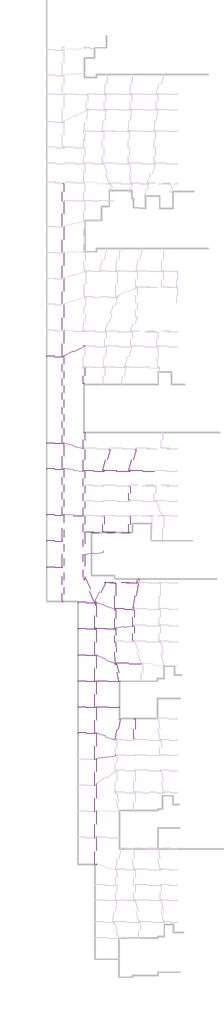
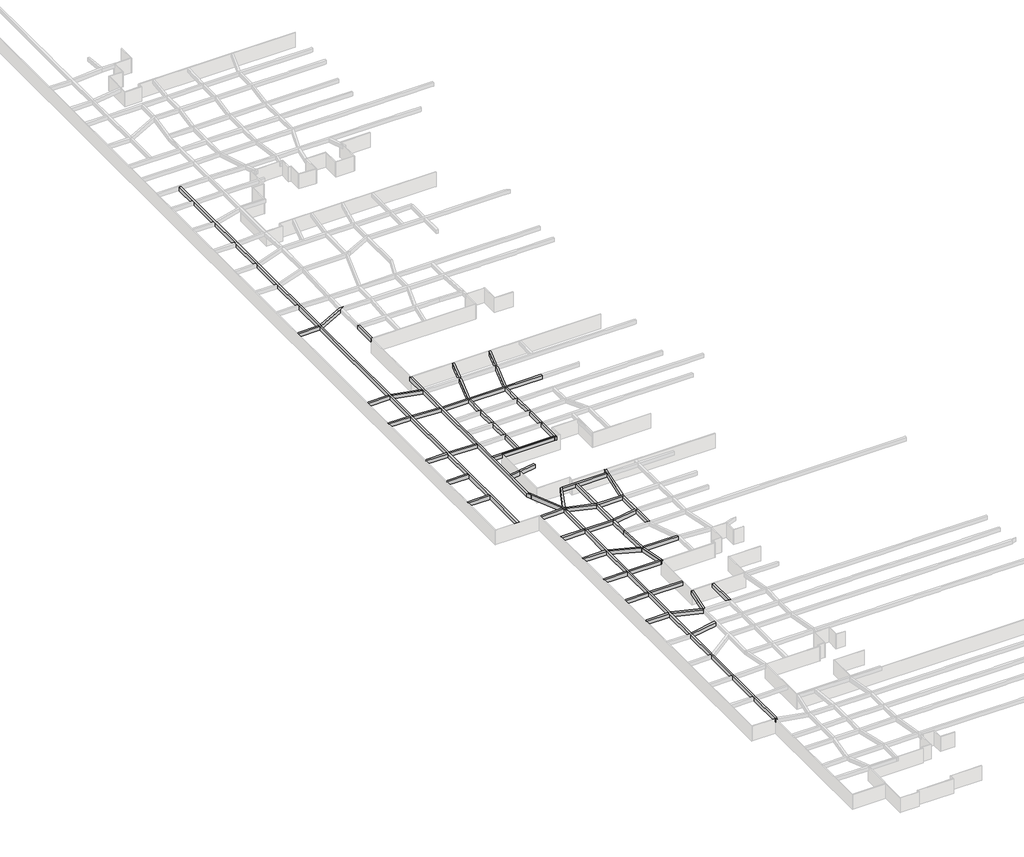
# One storey, part 14 of 45: 52 beams.
"""IFC4 building model written with IfcOpenShell, lengths in millimetres."""

from ifc_helpers import new_model, si_unit, frame, origin, place, context, project, spatial, polyline, outline, extrude, faceted_brep, element, save

model = new_model("IFC4")

# Units and contexts
model_context = context("Model", 3, world=origin())
ifc_project = project(units=[si_unit("LENGTHUNIT", "METRE", prefix="MILLI")], contexts=[model_context])

# Site, building, storey
site = spatial("IfcSite", under=ifc_project)
building = spatial("IfcBuilding", under=site)
storey = spatial("IfcBuildingStorey", under=building, Name="户型图", Elevation=0.0)

# Beams
placement = place(None, origin())
element("IfcBeam", 1, ObjectType="混凝土 - 矩形梁 : KL_beam", at=placement, inside=storey, context=model_context, shape_type="Brep", body=[
    faceted_brep([(-149959.8528414, -79527.7310375, 3300.0), (-150359.8528414, -79527.7310375, 3300.0), (-150359.8528414, -79527.7310375, 2500.0), (-149959.8528414, -79527.7310375, 2500.0), (-149959.8528414, -53780.5235569, 3300.0), (-149959.8528414, -53380.2797392, 3300.0), (-149959.8528414, -40042.1213562, 3300.0), (-149959.8528414, -39640.5934211, 3300.0), (-149959.8528414, -32335.6164347, 3300.0), (-149959.8528414, -31923.370983, 3300.0), (-149959.8528414, -6268.0099062, 3300.0), (-149959.8528414, -5819.0794111, 3300.0), (-149959.8528414, 1447.4441887, 3300.0), (-149959.8528414, 1847.6880064, 3300.0), (-149959.8528414, 9311.8916379, 3300.0), (-149959.8528414, 9734.9399104, 3300.0), (-149959.8528414, 17012.0067836, 3300.0), (-149959.8528414, 17435.0550561, 3300.0), (-149959.8528414, 24766.7995471, 3300.0), (-149959.8528414, 25167.5987199, 3300.0), (-149959.8528414, 32603.9353313, 3300.0), (-149959.8528414, 33020.0551056, 3300.0), (-149959.8528414, 40354.5502515, 3300.0), (-149959.8528414, 40754.5502515, 3300.0), (-149959.8528414, 45854.5502515, 3300.0), (-150359.8528414, 45854.5502515, 3300.0), (-150359.8528414, 40754.5502515, 3300.0), (-150359.8528414, 40354.5502515, 3300.0), (-150359.8528414, 32954.5502515, 3300.0), (-150359.8528414, 32554.5502515, 3300.0), (-150359.8528414, 25154.5502515, 3300.0), (-150359.8528414, 24754.5502515, 3300.0), (-150359.8528414, 17354.5502515, 3300.0), (-150359.8528414, 16954.5502515, 3300.0), (-150359.8528414, 9654.5502515, 3300.0), (-150359.8528414, 9254.5502515, 3300.0), (-150359.8528414, 1854.5502515, 3300.0), (-150359.8528414, 1454.5502515, 3300.0), (-150359.8528414, -5945.4497485, 3300.0), (-150359.8528414, -6345.4497485, 3300.0), (-150359.8528414, -31879.6281083, 3300.0), (-150359.8528414, -32279.6281083, 3300.0), (-150359.8528414, -39623.8596559, 3300.0), (-150359.8528414, -40023.8596559, 3300.0), (-150359.8528414, -53373.4174942, 3300.0), (-150359.8528414, -53773.4174942, 3300.0), (-150359.8528414, -61189.4871623, 3300.0), (-150359.8528414, -61589.4871623, 3300.0), (-150359.8528414, -69027.7310375, 3300.0), (-150359.8528414, -69427.7310375, 3300.0), (-150359.8528414, 45854.5502515, 2500.0), (-150359.8528414, 40754.5502515, 2500.0), (-150359.8528414, 40354.5502515, 2500.0), (-150359.8528414, 32954.5502515, 2500.0), (-150359.8528414, 32554.5502515, 2500.0), (-150359.8528414, 25154.5502515, 2500.0), (-150359.8528414, 24754.5502515, 2500.0), (-150359.8528414, 17354.5502515, 2500.0), (-150359.8528414, 16954.5502515, 2500.0), (-150359.8528414, 9654.5502515, 2500.0), (-150359.8528414, 9254.5502515, 2500.0), (-150359.8528414, 1854.5502515, 2500.0), (-150359.8528414, 1454.5502515, 2500.0), (-150359.8528414, -5945.4497485, 2500.0), (-150359.8528414, -6345.4497485, 2500.0), (-150359.8528414, -31879.6281083, 2500.0), (-150359.8528414, -32279.6281083, 2500.0), (-150359.8528414, -39623.8596559, 2500.0), (-150359.8528414, -40023.8596559, 2500.0), (-150359.8528414, -53373.4174942, 2500.0), (-150359.8528414, -53773.4174942, 2500.0), (-150359.8528414, -61189.4871623, 2500.0), (-150359.8528414, -61589.4871623, 2500.0), (-150359.8528414, -69027.7310375, 2500.0), (-150359.8528414, -69427.7310375, 2500.0), (-149959.8528414, 45854.5502515, 2500.0), (-149959.8528414, 40754.5502515, 2500.0), (-149959.8528414, 40354.5502515, 2500.0), (-149959.8528414, 33020.0551056, 2500.0), (-149959.8528414, 32603.9353313, 2500.0), (-149959.8528414, 25167.5987199, 2500.0), (-149959.8528414, 24766.7995471, 2500.0), (-149959.8528414, 17435.0550561, 2500.0), (-149959.8528414, 17012.0067836, 2500.0), (-149959.8528414, 9734.9399104, 2500.0), (-149959.8528414, 9311.8916379, 2500.0), (-149959.8528414, 1847.6880064, 2500.0), (-149959.8528414, 1447.4441887, 2500.0), (-149959.8528414, -5819.0794111, 2500.0), (-149959.8528414, -6268.0099062, 2500.0), (-149959.8528414, -31923.370983, 2500.0), (-149959.8528414, -32335.6164347, 2500.0), (-149959.8528414, -39640.5934211, 2500.0), (-149959.8528414, -40042.1213562, 2500.0), (-149959.8528414, -53380.2797392, 2500.0), (-149959.8528414, -53780.5235569, 2500.0)], [[[0, 1, 2, 3]], [[1, 0, 4, 5, 6, 7, 8, 9, 10, 11, 12, 13, 14, 15, 16, 17, 18, 19, 20, 21, 22, 23, 24, 25, 26, 27, 28, 29, 30, 31, 32, 33, 34, 35, 36, 37, 38, 39, 40, 41, 42, 43, 44, 45, 46, 47, 48, 49]], [[2, 1, 49, 48, 47, 46, 45, 44, 43, 42, 41, 40, 39, 38, 37, 36, 35, 34, 33, 32, 31, 30, 29, 28, 27, 26, 25, 50, 51, 52, 53, 54, 55, 56, 57, 58, 59, 60, 61, 62, 63, 64, 65, 66, 67, 68, 69, 70, 71, 72, 73, 74]], [[3, 2, 74, 73, 72, 71, 70, 69, 68, 67, 66, 65, 64, 63, 62, 61, 60, 59, 58, 57, 56, 55, 54, 53, 52, 51, 50, 75, 76, 77, 78, 79, 80, 81, 82, 83, 84, 85, 86, 87, 88, 89, 90, 91, 92, 93, 94, 95]], [[0, 3, 95, 94, 93, 92, 91, 90, 89, 88, 87, 86, 85, 84, 83, 82, 81, 80, 79, 78, 77, 76, 75, 24, 23, 22, 21, 20, 19, 18, 17, 16, 15, 14, 13, 12, 11, 10, 9, 8, 7, 6, 5, 4]], [[25, 24, 75, 50]]]),
])
element("IfcBeam", 2, ObjectType="混凝土 - 矩形梁 : KL_beam", at=placement, inside=storey, context=model_context, shape_type="SweptSolid", body=[
    extrude(outline(polyline([(-155040.1872489, -6345.4497485), (-155040.1872489, -5945.4497485), (-150359.8528414, -5945.4497485), (-150359.8528414, -6345.4497485), (-155040.1872489, -6345.4497485)])), frame((0.0, 0.0, 2500.0), z_axis=(0.0, 0.0, 1.0), x_axis=(1.0, 0.0, 0.0)), (0.0, 0.0, 1.0), 800.0),
])
element("IfcBeam", 3, ObjectType="混凝土 - 矩形梁 : KL_beam", at=placement, inside=storey, context=model_context, shape_type="Brep", body=[
    faceted_brep([(-143362.5840071, -2906.533538, 3300.0), (-143704.0852782, -2906.533538, 3300.0), (-144104.0852782, -2906.533538, 3300.0), (-144243.659713, -2906.533538, 3300.0), (-149959.8528414, -5819.0794111, 3300.0), (-149959.8528414, -6268.0099062, 3300.0), (-144147.6282093, -3306.533538, 3300.0), (-143362.5840071, -2906.533538, 2500.0), (-149959.8528414, -6268.0099062, 2500.0), (-144147.6282093, -3306.533538, 2500.0), (-144243.659713, -2906.533538, 2500.0), (-144104.0852782, -2906.533538, 2500.0), (-143704.0852782, -2906.533538, 2500.0), (-149959.8528414, -5819.0794111, 2500.0)], [[[0, 1, 2, 3, 4, 5, 6]], [[7, 0, 6, 5, 8, 9]], [[10, 11, 12, 7, 9, 8, 13]], [[3, 10, 13, 4]], [[5, 4, 13, 8]], [[3, 2, 1, 0, 7, 12, 11, 10]]]),
])
element("IfcBeam", 4, ObjectType="混凝土 - 矩形梁 : KL_beam", at=placement, inside=storey, context=model_context, shape_type="SweptSolid", body=[
    extrude(outline(polyline([(-143704.0852782, -14343.8680223), (-144104.0852782, -14343.8680223), (-144104.0852782, -9543.8680223), (-143704.0852782, -9543.8680223), (-143704.0852782, -14343.8680223)])), frame((0.0, 0.0, 2500.0), z_axis=(0.0, 0.0, 1.0), x_axis=(1.0, 0.0, 0.0)), (0.0, 0.0, 1.0), 800.0),
])
element("IfcBeam", 5, ObjectType="混凝土 - 矩形梁 : KL_beam", at=placement, inside=storey, context=model_context, shape_type="Brep", body=[
    faceted_brep([(-122515.2422867, -40570.1922876, 3300.0), (-122515.2422867, -40170.1922876, 3300.0), (-130022.2070751, -40170.1922876, 3300.0), (-130438.3268494, -40170.1922876, 3300.0), (-137822.2070751, -40170.1922876, 3300.0), (-138238.3268494, -40170.1922876, 3300.0), (-143687.6160394, -40170.1922876, 3300.0), (-143687.6160394, -40570.1922876, 3300.0), (-138287.6160394, -40570.1922876, 3300.0), (-137887.6160394, -40570.1922876, 3300.0), (-130487.6160394, -40570.1922876, 3300.0), (-130087.6160394, -40570.1922876, 3300.0), (-122515.2422867, -40570.1922876, 2500.0), (-143687.6160394, -40570.1922876, 2500.0), (-138287.6160394, -40570.1922876, 2500.0), (-137887.6160394, -40570.1922876, 2500.0), (-130487.6160394, -40570.1922876, 2500.0), (-130087.6160394, -40570.1922876, 2500.0), (-122515.2422867, -40170.1922876, 2500.0), (-143687.6160394, -40170.1922876, 2500.0), (-138238.3268494, -40170.1922876, 2500.0), (-137822.2070751, -40170.1922876, 2500.0), (-130438.3268494, -40170.1922876, 2500.0), (-130022.2070751, -40170.1922876, 2500.0)], [[[0, 1, 2, 3, 4, 5, 6, 7, 8, 9, 10, 11]], [[12, 0, 11, 10, 9, 8, 7, 13, 14, 15, 16, 17]], [[18, 12, 17, 16, 15, 14, 13, 19, 20, 21, 22, 23]], [[1, 18, 23, 22, 21, 20, 19, 6, 5, 4, 3, 2]], [[1, 0, 12, 18]], [[7, 6, 19, 13]]]),
])
element("IfcBeam", 6, ObjectType="混凝土 - 矩形梁 : KL_beam", at=placement, inside=storey, context=model_context, shape_type="SweptSolid", body=[
    extrude(outline(polyline([(-144087.6160394, -33387.4840571), (-144087.6160394, -33799.7295088), (-149959.8528414, -32335.6164347), (-149959.8528414, -31923.370983), (-144087.6160394, -33387.4840571)])), frame((0.0, 0.0, 2500.0), z_axis=(0.0, 0.0, 1.0), x_axis=(1.0, 0.0, 0.0)), (0.0, 0.0, 1.0), 800.0),
])
element("IfcBeam", 7, ObjectType="混凝土 - 矩形梁 : KL_beam", at=placement, inside=storey, context=model_context, shape_type="SweptSolid", body=[
    extrude(outline(polyline([(-155040.1872489, -32279.6281083), (-155040.1872489, -31879.6281083), (-150359.8528414, -31879.6281083), (-150359.8528414, -32279.6281083), (-155040.1872489, -32279.6281083)])), frame((0.0, 0.0, 2500.0), z_axis=(0.0, 0.0, 1.0), x_axis=(1.0, 0.0, 0.0)), (0.0, 0.0, 1.0), 800.0),
])
element("IfcBeam", 8, ObjectType="混凝土 - 矩形梁 : KL_beam", at=placement, inside=storey, context=model_context, shape_type="SweptSolid", body=[
    extrude(outline(polyline([(-144087.6160394, -40154.3475708), (-144087.6160394, -40555.8755059), (-149959.8528414, -40042.1213562), (-149959.8528414, -39640.5934211), (-144087.6160394, -40154.3475708)])), frame((0.0, 0.0, 2500.0), z_axis=(0.0, 0.0, 1.0), x_axis=(1.0, 0.0, 0.0)), (0.0, 0.0, 1.0), 800.0),
])
element("IfcBeam", 9, ObjectType="混凝土 - 矩形梁 : KL_beam", at=placement, inside=storey, context=model_context, shape_type="SweptSolid", body=[
    extrude(outline(polyline([(-155040.1872489, -40023.8596559), (-155040.1872489, -39623.8596559), (-150359.8528414, -39623.8596559), (-150359.8528414, -40023.8596559), (-155040.1872489, -40023.8596559)])), frame((0.0, 0.0, 2500.0), z_axis=(0.0, 0.0, 1.0), x_axis=(1.0, 0.0, 0.0)), (0.0, 0.0, 1.0), 800.0),
])
element("IfcBeam", 10, ObjectType="混凝土 - 矩形梁 : KL_beam", at=placement, inside=storey, context=model_context, shape_type="SweptSolid", body=[
    extrude(outline(polyline([(-149959.8528414, -53780.5235569), (-149959.8528414, -53380.2797392), (-144087.6160394, -53585.342767), (-144087.6160394, -53985.5865847), (-149959.8528414, -53780.5235569)])), frame((0.0, 0.0, 2500.0), z_axis=(0.0, 0.0, 1.0), x_axis=(1.0, 0.0, 0.0)), (0.0, 0.0, 1.0), 800.0),
])
element("IfcBeam", 11, ObjectType="混凝土 - 矩形梁 : KL_beam", at=placement, inside=storey, context=model_context, shape_type="SweptSolid", body=[
    extrude(outline(polyline([(-155040.1872489, -53773.4174942), (-155040.1872489, -53373.4174942), (-150359.8528414, -53373.4174942), (-150359.8528414, -53773.4174942), (-155040.1872489, -53773.4174942)])), frame((0.0, 0.0, 2500.0), z_axis=(0.0, 0.0, 1.0), x_axis=(1.0, 0.0, 0.0)), (0.0, 0.0, 1.0), 800.0),
])
element("IfcBeam", 12, ObjectType="混凝土 - 矩形梁 : KL_beam", at=placement, inside=storey, context=model_context, shape_type="SweptSolid", body=[
    extrude(outline(polyline([(-155040.1872489, -61589.4871623), (-155040.1872489, -61189.4871623), (-150359.8528414, -61189.4871623), (-150359.8528414, -61589.4871623), (-155040.1872489, -61589.4871623)])), frame((0.0, 0.0, 2500.0), z_axis=(0.0, 0.0, 1.0), x_axis=(1.0, 0.0, 0.0)), (0.0, 0.0, 1.0), 800.0),
])
element("IfcBeam", 13, ObjectType="混凝土 - 矩形梁 : KL_beam", at=placement, inside=storey, context=model_context, shape_type="SweptSolid", body=[
    extrude(outline(polyline([(-155040.1872489, -69427.7310375), (-155040.1872489, -69027.7310375), (-150359.8528414, -69027.7310375), (-150359.8528414, -69427.7310375), (-155040.1872489, -69427.7310375)])), frame((0.0, 0.0, 2500.0), z_axis=(0.0, 0.0, 1.0), x_axis=(1.0, 0.0, 0.0)), (0.0, 0.0, 1.0), 800.0),
])
element("IfcBeam", 14, ObjectType="混凝土 - 矩形梁 : KL_beam", at=placement, inside=storey, context=model_context, shape_type="Brep", body=[
    faceted_brep([(-143687.6160394, -28841.7316236, 3300.0), (-143687.6160394, -28841.7316236, 2500.0), (-144087.6160394, -28841.7316236, 2500.0), (-144087.6160394, -28841.7316236, 3300.0), (-144087.6160394, -33387.4840571, 3300.0), (-144087.6160394, -33799.7295088, 3300.0), (-144087.6160394, -40154.3475708, 3300.0), (-144087.6160394, -40555.8755059, 3300.0), (-144087.6160394, -53585.342767, 3300.0), (-144087.6160394, -53985.5865847, 3300.0), (-144087.6160394, -72184.2429359, 3300.0), (-143687.6160394, -73082.6576455, 3300.0), (-143687.6160394, -72099.2203112, 3300.0), (-143687.6160394, -65809.5515498, 3300.0), (-143687.6160394, -65403.3809051, 3300.0), (-143687.6160394, -58989.4871623, 3300.0), (-143687.6160394, -58589.4871623, 3300.0), (-143687.6160394, -53989.4871623, 3300.0), (-143687.6160394, -53589.4871623, 3300.0), (-143687.6160394, -49549.7368283, 3300.0), (-143687.6160394, -49149.7368283, 3300.0), (-143687.6160394, -44984.7380181, 3300.0), (-143687.6160394, -44584.7380181, 3300.0), (-143687.6160394, -40570.1922876, 3300.0), (-143687.6160394, -40170.1922876, 3300.0), (-143687.6160394, -33842.9557231, 3300.0), (-143687.6160394, -33442.9557231, 3300.0), (-144087.6160394, -33387.4840571, 2500.0), (-144087.6160394, -33799.7295088, 2500.0), (-144087.6160394, -40154.3475708, 2500.0), (-144087.6160394, -40555.8755059, 2500.0), (-144087.6160394, -53585.342767, 2500.0), (-144087.6160394, -53985.5865847, 2500.0), (-144087.6160394, -72184.2429359, 2500.0), (-143687.6160394, -33442.9557231, 2500.0), (-143687.6160394, -33842.9557231, 2500.0), (-143687.6160394, -40170.1922876, 2500.0), (-143687.6160394, -40570.1922876, 2500.0), (-143687.6160394, -44584.7380181, 2500.0), (-143687.6160394, -44984.7380181, 2500.0), (-143687.6160394, -49149.7368283, 2500.0), (-143687.6160394, -49549.7368283, 2500.0), (-143687.6160394, -53589.4871623, 2500.0), (-143687.6160394, -53989.4871623, 2500.0), (-143687.6160394, -58589.4871623, 2500.0), (-143687.6160394, -58989.4871623, 2500.0), (-143687.6160394, -65403.3809051, 2500.0), (-143687.6160394, -65809.5515498, 2500.0), (-143687.6160394, -72099.2203112, 2500.0), (-143687.6160394, -73082.6576455, 2500.0)], [[[0, 1, 2, 3]], [[0, 3, 4, 5, 6, 7, 8, 9, 10, 11, 12, 13, 14, 15, 16, 17, 18, 19, 20, 21, 22, 23, 24, 25, 26]], [[3, 2, 27, 28, 29, 30, 31, 32, 33, 10, 9, 8, 7, 6, 5, 4]], [[2, 1, 34, 35, 36, 37, 38, 39, 40, 41, 42, 43, 44, 45, 46, 47, 48, 49, 33, 32, 31, 30, 29, 28, 27]], [[1, 0, 26, 25, 24, 23, 22, 21, 20, 19, 18, 17, 16, 15, 14, 13, 12, 11, 49, 48, 47, 46, 45, 44, 43, 42, 41, 40, 39, 38, 37, 36, 35, 34]], [[11, 10, 33, 49]]]),
])
element("IfcBeam", 15, ObjectType="混凝土 - 矩形梁 : KL_beam", at=placement, inside=storey, context=model_context, shape_type="Brep", body=[
    faceted_brep([(-140271.0282376, -80756.4394897, 3300.0), (-140271.0282376, -80088.1741567, 3300.0), (-140271.0282376, -79773.0021554, 3300.0), (-140324.9318597, -79651.9326379, 3300.0), (-140466.6372594, -79333.6570992, 3300.0), (-143687.6160394, -72099.2203112, 3300.0), (-143687.6160394, -73082.6576455, 3300.0), (-140778.9001436, -79615.7405122, 3300.0), (-140671.0282376, -79858.0247801, 3300.0), (-140271.0282376, -80756.4394897, 2500.0), (-143687.6160394, -73082.6576455, 2500.0), (-140778.9001436, -79615.7405122, 2500.0), (-140671.0282376, -79858.0247801, 2500.0), (-140271.0282376, -79773.0021554, 2500.0), (-140271.0282376, -80088.1741567, 2500.0), (-143687.6160394, -72099.2203112, 2500.0), (-140466.6372594, -79333.6570992, 2500.0), (-140324.9318597, -79651.9326379, 2500.0)], [[[0, 1, 2, 3, 4, 5, 6, 7, 8]], [[9, 0, 8, 7, 6, 10, 11, 12]], [[13, 14, 9, 12, 11, 10, 15, 16, 17]], [[2, 13, 17, 16, 15, 5, 4, 3]], [[6, 5, 15, 10]], [[2, 1, 0, 9, 14, 13]]]),
])
element("IfcBeam", 16, ObjectType="混凝土 - 矩形梁 : KL_beam", at=placement, inside=storey, context=model_context, shape_type="SweptSolid", body=[
    extrude(outline(polyline([(-138287.6160394, -40570.1922876), (-137887.6160394, -40570.1922876), (-137887.6160394, -44584.7380181), (-138287.6160394, -44584.7380181), (-138287.6160394, -40570.1922876)])), frame((0.0, 0.0, 2500.0), z_axis=(0.0, 0.0, 1.0), x_axis=(1.0, 0.0, 0.0)), (0.0, 0.0, 1.0), 800.0),
    extrude(outline(polyline([(-138287.6160394, -44984.7380181), (-137887.6160394, -44984.7380181), (-137887.6160394, -49149.7368283), (-138287.6160394, -49149.7368283), (-138287.6160394, -44984.7380181)])), frame((0.0, 0.0, 2500.0), z_axis=(0.0, 0.0, 1.0), x_axis=(1.0, 0.0, 0.0)), (0.0, 0.0, 1.0), 800.0),
    extrude(outline(polyline([(-138287.6160394, -49549.7368283), (-137887.6160394, -49549.7368283), (-137887.6160394, -53589.4871623), (-138287.6160394, -53589.4871623), (-138287.6160394, -49549.7368283)])), frame((0.0, 0.0, 2500.0), z_axis=(0.0, 0.0, 1.0), x_axis=(1.0, 0.0, 0.0)), (0.0, 0.0, 1.0), 800.0),
    extrude(outline(polyline([(-138287.6160394, -53989.4871623), (-137887.6160394, -53989.4871623), (-137887.6160394, -58589.4871623), (-138287.6160394, -58589.4871623), (-138287.6160394, -53989.4871623)])), frame((0.0, 0.0, 2500.0), z_axis=(0.0, 0.0, 1.0), x_axis=(1.0, 0.0, 0.0)), (0.0, 0.0, 1.0), 800.0),
])
element("IfcBeam", 17, ObjectType="混凝土 - 矩形梁 : KL_beam", at=placement, inside=storey, context=model_context, shape_type="SweptSolid", body=[
    extrude(outline(polyline([(-134969.1006355, -28769.0455688), (-134584.5959571, -28879.3005111), (-135893.2030313, -33442.9557231), (-136309.3228056, -33442.9557231), (-134969.1006355, -28769.0455688)])), frame((0.0, 0.0, 2500.0), z_axis=(0.0, 0.0, 1.0), x_axis=(1.0, 0.0, 0.0)), (0.0, 0.0, 1.0), 800.0),
    extrude(outline(polyline([(-136424.0209599, -33842.9557231), (-136007.9011856, -33842.9557231), (-137822.2070751, -40170.1922876), (-138238.3268494, -40170.1922876), (-136424.0209599, -33842.9557231)])), frame((0.0, 0.0, 2500.0), z_axis=(0.0, 0.0, 1.0), x_axis=(1.0, 0.0, 0.0)), (0.0, 0.0, 1.0), 800.0),
])
element("IfcBeam", 18, ObjectType="混凝土 - 矩形梁 : KL_beam", at=placement, inside=storey, context=model_context, shape_type="SweptSolid", body=[
    extrude(outline(polyline([(-127169.1006355, -28769.0455688), (-126784.5959571, -28879.3005111), (-128093.2030313, -33442.9557231), (-128509.3228056, -33442.9557231), (-127169.1006355, -28769.0455688)])), frame((0.0, 0.0, 2500.0), z_axis=(0.0, 0.0, 1.0), x_axis=(1.0, 0.0, 0.0)), (0.0, 0.0, 1.0), 800.0),
    extrude(outline(polyline([(-128624.0209599, -33842.9557231), (-128207.9011856, -33842.9557231), (-130022.2070751, -40170.1922876), (-130438.3268494, -40170.1922876), (-128624.0209599, -33842.9557231)])), frame((0.0, 0.0, 2500.0), z_axis=(0.0, 0.0, 1.0), x_axis=(1.0, 0.0, 0.0)), (0.0, 0.0, 1.0), 800.0),
])
element("IfcBeam", 19, ObjectType="混凝土 - 矩形梁 : KL_beam", at=placement, inside=storey, context=model_context, shape_type="SweptSolid", body=[
    extrude(outline(polyline([(-130487.6160394, -40570.1922876), (-130087.6160394, -40570.1922876), (-130087.6160394, -44584.7380181), (-130487.6160394, -44584.7380181), (-130487.6160394, -40570.1922876)])), frame((0.0, 0.0, 2500.0), z_axis=(0.0, 0.0, 1.0), x_axis=(1.0, 0.0, 0.0)), (0.0, 0.0, 1.0), 800.0),
    extrude(outline(polyline([(-130087.6160394, -53589.4871623), (-130487.6160394, -53589.4871623), (-130487.6160394, -49549.7368283), (-130087.6160394, -49549.7368283), (-130087.6160394, -53589.4871623)])), frame((0.0, 0.0, 2500.0), z_axis=(0.0, 0.0, 1.0), x_axis=(1.0, 0.0, 0.0)), (0.0, 0.0, 1.0), 800.0),
    extrude(outline(polyline([(-130487.6160394, -44984.7380181), (-130087.6160394, -44984.7380181), (-130087.6160394, -49149.7368283), (-130487.6160394, -49149.7368283), (-130487.6160394, -44984.7380181)])), frame((0.0, 0.0, 2500.0), z_axis=(0.0, 0.0, 1.0), x_axis=(1.0, 0.0, 0.0)), (0.0, 0.0, 1.0), 800.0),
])
element("IfcBeam", 20, ObjectType="混凝土 - 矩形梁 : KL_beam", at=placement, inside=storey, context=model_context, shape_type="Brep", body=[
    faceted_brep([(-130487.6160394, -58989.4871623, 3300.0), (-130087.6160394, -58989.4871623, 3300.0), (-130087.6160394, -53989.4871623, 3300.0), (-130487.6160394, -53989.4871623, 3300.0), (-130487.6160394, -58589.4871623, 3300.0), (-130487.6160394, -58989.4871623, 2500.0), (-130487.6160394, -53989.4871623, 2500.0), (-130487.6160394, -58589.4871623, 2500.0), (-130087.6160394, -58989.4871623, 2500.0), (-130087.6160394, -53989.4871623, 2500.0)], [[[0, 1, 2, 3, 4]], [[5, 0, 4, 3, 6, 7]], [[8, 5, 7, 6, 9]], [[1, 8, 9, 2]], [[3, 2, 9, 6]], [[1, 0, 5, 8]]]),
])
element("IfcBeam", 21, ObjectType="混凝土 - 矩形梁 : KL_beam", at=placement, inside=storey, context=model_context, shape_type="Brep", body=[
    faceted_brep([(-128818.6286131, -81886.7344834, 3300.0), (-128818.6286131, -81486.7344834, 3300.0), (-129189.4447502, -81486.7344834, 3300.0), (-134318.6286131, -81486.7344834, 3300.0), (-134488.0377959, -81486.7344834, 3300.0), (-134718.6286131, -81486.7344834, 3300.0), (-134718.6286131, -81833.5464328, 3300.0), (-134718.6286131, -81886.7344834, 3300.0), (-134318.6286131, -81886.7344834, 3300.0), (-129218.6286131, -81886.7344834, 3300.0), (-128818.6286131, -81886.7344834, 2500.0), (-134718.6286131, -81886.7344834, 2500.0), (-134318.6286131, -81886.7344834, 2500.0), (-129218.6286131, -81886.7344834, 2500.0), (-128818.6286131, -81486.7344834, 2500.0), (-134718.6286131, -81833.5464328, 2500.0), (-134718.6286131, -81486.7344834, 2500.0), (-134488.0377959, -81486.7344834, 2500.0), (-134318.6286131, -81486.7344834, 2500.0), (-129189.4447502, -81486.7344834, 2500.0)], [[[0, 1, 2, 3, 4, 5, 6, 7, 8, 9]], [[10, 0, 9, 8, 7, 11, 12, 13]], [[14, 10, 13, 12, 11, 15, 16, 17, 18, 19]], [[1, 14, 19, 18, 17, 16, 5, 4, 3, 2]], [[1, 0, 10, 14]], [[7, 6, 5, 16, 15, 11]]]),
])
element("IfcBeam", 22, ObjectType="混凝土 - 矩形梁 : KL_beam", at=placement, inside=storey, context=model_context, shape_type="Brep", body=[
    faceted_brep([(-129218.6286131, -86925.0852019, 3300.0), (-129001.1308804, -86886.7344834, 3300.0), (-128818.6286131, -86854.5544096, 3300.0), (-128818.6286131, -86486.7344834, 3300.0), (-128818.6286131, -81886.7344834, 3300.0), (-129218.6286131, -81886.7344834, 3300.0), (-129218.6286131, -86518.9145571, 3300.0), (-129218.6286131, -86925.0852019, 2500.0), (-129218.6286131, -81886.7344834, 2500.0), (-129218.6286131, -86518.9145571, 2500.0), (-128818.6286131, -86854.5544096, 2500.0), (-129001.1308804, -86886.7344834, 2500.0), (-128818.6286131, -81886.7344834, 2500.0), (-128818.6286131, -86486.7344834, 2500.0)], [[[0, 1, 2, 3, 4, 5, 6]], [[7, 0, 6, 5, 8, 9]], [[10, 11, 7, 9, 8, 12, 13]], [[2, 10, 13, 12, 4, 3]], [[5, 4, 12, 8]], [[2, 1, 0, 7, 11, 10]]]),
])
element("IfcBeam", 23, ObjectType="混凝土 - 矩形梁 : KL_beam", at=placement, inside=storey, context=model_context, shape_type="Brep", body=[
    faceted_brep([(-134452.5689874, -87441.7994605, 3300.0), (-134417.573522, -87841.7994605, 3300.0), (-134318.6286131, -87824.3528035, 3300.0), (-129218.6286131, -86925.0852019, 3300.0), (-129218.6286131, -86518.9145571, 3300.0), (-134318.6286131, -87418.1821587, 3300.0), (-134452.5689874, -87441.7994605, 2500.0), (-129218.6286131, -86518.9145571, 2500.0), (-134318.6286131, -87418.1821587, 2500.0), (-134417.573522, -87841.7994605, 2500.0), (-129218.6286131, -86925.0852019, 2500.0), (-134318.6286131, -87824.3528035, 2500.0)], [[[0, 1, 2, 3, 4, 5]], [[6, 0, 5, 4, 7, 8]], [[9, 6, 8, 7, 10, 11]], [[1, 9, 11, 10, 3, 2]], [[4, 3, 10, 7]], [[1, 0, 6, 9]]]),
])
element("IfcBeam", 24, ObjectType="混凝土 - 矩形梁 : KL_beam", at=placement, inside=storey, context=model_context, shape_type="Brep", body=[
    faceted_brep([(-134417.573522, -87841.7994605, 3300.0), (-134452.5689874, -87441.7994605, 3300.0), (-134718.6286131, -87441.7994605, 3300.0), (-140271.0282376, -87441.7994605, 3300.0), (-140635.0712547, -87441.7994605, 3300.0), (-140635.0712547, -87841.7994605, 3300.0), (-140235.0712547, -87841.7994605, 3300.0), (-134718.6286131, -87841.7994605, 3300.0), (-134452.5689874, -87441.7994605, 2500.0), (-134718.6286131, -87441.7994605, 2500.0), (-140271.0282376, -87441.7994605, 2500.0), (-140635.0712547, -87441.7994605, 2500.0), (-134417.573522, -87841.7994605, 2500.0), (-134718.6286131, -87841.7994605, 2500.0), (-140235.0712547, -87841.7994605, 2500.0), (-140635.0712547, -87841.7994605, 2500.0)], [[[0, 1, 2, 3, 4, 5, 6, 7]], [[1, 8, 9, 10, 11, 4, 3, 2]], [[8, 12, 13, 14, 15, 11, 10, 9]], [[12, 0, 7, 6, 5, 15, 14, 13]], [[0, 12, 8, 1]], [[5, 4, 11, 15]]]),
])
element("IfcBeam", 25, ObjectType="混凝土 - 矩形梁 : KL_beam", at=placement, inside=storey, context=model_context, shape_type="SweptSolid", body=[
    extrude(outline(polyline([(-134718.6286131, -81886.7344834), (-134318.6286131, -81886.7344834), (-134318.6286131, -87418.1821587), (-134452.5689874, -87441.7994605), (-134718.6286131, -87441.7994605), (-134718.6286131, -81886.7344834)])), frame((0.0, 0.0, 2500.0), z_axis=(0.0, 0.0, 1.0), x_axis=(1.0, 0.0, 0.0)), (0.0, 0.0, 1.0), 800.0),
])
element("IfcBeam", 26, ObjectType="混凝土 - 矩形梁 : KL_beam", at=placement, inside=storey, context=model_context, shape_type="Brep", body=[
    faceted_brep([(-134417.573522, -87841.7994605, 3300.0), (-134718.6286131, -87841.7994605, 3300.0), (-134718.6286131, -91641.7669719, 3300.0), (-134711.7663681, -91641.7669719, 3300.0), (-134318.6286131, -91641.7669719, 3300.0), (-134318.6286131, -91241.7669719, 3300.0), (-134318.6286131, -87824.3528035, 3300.0), (-134718.6286131, -87841.7994605, 2500.0), (-134718.6286131, -91641.7669719, 2500.0), (-134417.573522, -87841.7994605, 2500.0), (-134318.6286131, -87824.3528035, 2500.0), (-134318.6286131, -91241.7669719, 2500.0), (-134318.6286131, -91641.7669719, 2500.0), (-134711.7663681, -91641.7669719, 2500.0)], [[[0, 1, 2, 3, 4, 5, 6]], [[1, 7, 8, 2]], [[7, 9, 10, 11, 12, 13, 8]], [[10, 6, 5, 4, 12, 11]], [[1, 0, 9, 7]], [[0, 6, 10, 9]], [[4, 3, 2, 8, 13, 12]]]),
])
element("IfcBeam", 27, ObjectType="混凝土 - 矩形梁 : KL_beam", at=placement, inside=storey, context=model_context, shape_type="Brep", body=[
    faceted_brep([(-140635.0712547, -158399.1295185, 3300.0), (-140235.0712547, -158496.0420414, 3300.0), (-140235.0712547, -158084.4694025, 3300.0), (-140235.0712547, -150329.5553627, 3300.0), (-140235.0712547, -149929.5553627, 3300.0), (-140235.0712547, -142522.6839278, 3300.0), (-140235.0712547, -142122.4401101, 3300.0), (-140235.0712547, -134607.1099192, 3300.0), (-140235.0712547, -134112.6827282, 3300.0), (-140235.0712547, -126910.8224065, 3300.0), (-140235.0712547, -126503.1705503, 3300.0), (-140235.0712547, -119155.7020829, 3300.0), (-140235.0712547, -118732.7040614, 3300.0), (-140235.0712547, -111375.3373066, 3300.0), (-140235.0712547, -110975.3373066, 3300.0), (-140235.0712547, -103575.0953667, 3300.0), (-140235.0712547, -103175.0953667, 3300.0), (-140235.0712547, -95870.908911, 3300.0), (-140235.0712547, -95440.0063093, 3300.0), (-140235.0712547, -87841.7994605, 3300.0), (-140635.0712547, -87841.7994605, 3300.0), (-140635.0712547, -95375.3373066, 3300.0), (-140635.0712547, -95775.3373066, 3300.0), (-140635.0712547, -103175.3373066, 3300.0), (-140635.0712547, -103575.3373066, 3300.0), (-140635.0712547, -110975.3373066, 3300.0), (-140635.0712547, -111375.3373066, 3300.0), (-140635.0712547, -118675.3373066, 3300.0), (-140635.0712547, -119075.3373066, 3300.0), (-140635.0712547, -126546.3745528, 3300.0), (-140635.0712547, -126946.3745528, 3300.0), (-140635.0712547, -134305.27306, 3300.0), (-140635.0712547, -134705.27306, 3300.0), (-140635.0712547, -142129.5553627, 3300.0), (-140635.0712547, -142529.5553627, 3300.0), (-140635.0712547, -149929.5553627, 3300.0), (-140635.0712547, -150329.5553627, 3300.0), (-140635.0712547, -158399.1295185, 2500.0), (-140635.0712547, -87841.7994605, 2500.0), (-140635.0712547, -95375.3373066, 2500.0), (-140635.0712547, -95775.3373066, 2500.0), (-140635.0712547, -103175.3373066, 2500.0), (-140635.0712547, -103575.3373066, 2500.0), (-140635.0712547, -110975.3373066, 2500.0), (-140635.0712547, -111375.3373066, 2500.0), (-140635.0712547, -118675.3373066, 2500.0), (-140635.0712547, -119075.3373066, 2500.0), (-140635.0712547, -126546.3745528, 2500.0), (-140635.0712547, -126946.3745528, 2500.0), (-140635.0712547, -134305.27306, 2500.0), (-140635.0712547, -134705.27306, 2500.0), (-140635.0712547, -142129.5553627, 2500.0), (-140635.0712547, -142529.5553627, 2500.0), (-140635.0712547, -149929.5553627, 2500.0), (-140635.0712547, -150329.5553627, 2500.0), (-140235.0712547, -158496.0420414, 2500.0), (-140235.0712547, -87841.7994605, 2500.0), (-140235.0712547, -95440.0063093, 2500.0), (-140235.0712547, -95870.908911, 2500.0), (-140235.0712547, -103175.0953667, 2500.0), (-140235.0712547, -103575.0953667, 2500.0), (-140235.0712547, -110975.3373066, 2500.0), (-140235.0712547, -111375.3373066, 2500.0), (-140235.0712547, -118732.7040614, 2500.0), (-140235.0712547, -119155.7020829, 2500.0), (-140235.0712547, -126503.1705503, 2500.0), (-140235.0712547, -126910.8224065, 2500.0), (-140235.0712547, -134112.6827282, 2500.0), (-140235.0712547, -134607.1099192, 2500.0), (-140235.0712547, -142122.4401101, 2500.0), (-140235.0712547, -142522.6839278, 2500.0), (-140235.0712547, -149929.5553627, 2500.0), (-140235.0712547, -150329.5553627, 2500.0), (-140235.0712547, -158084.4694025, 2500.0)], [[[0, 1, 2, 3, 4, 5, 6, 7, 8, 9, 10, 11, 12, 13, 14, 15, 16, 17, 18, 19, 20, 21, 22, 23, 24, 25, 26, 27, 28, 29, 30, 31, 32, 33, 34, 35, 36]], [[37, 0, 36, 35, 34, 33, 32, 31, 30, 29, 28, 27, 26, 25, 24, 23, 22, 21, 20, 38, 39, 40, 41, 42, 43, 44, 45, 46, 47, 48, 49, 50, 51, 52, 53, 54]], [[55, 37, 54, 53, 52, 51, 50, 49, 48, 47, 46, 45, 44, 43, 42, 41, 40, 39, 38, 56, 57, 58, 59, 60, 61, 62, 63, 64, 65, 66, 67, 68, 69, 70, 71, 72, 73]], [[1, 55, 73, 72, 71, 70, 69, 68, 67, 66, 65, 64, 63, 62, 61, 60, 59, 58, 57, 56, 19, 18, 17, 16, 15, 14, 13, 12, 11, 10, 9, 8, 7, 6, 5, 4, 3, 2]], [[20, 19, 56, 38]], [[1, 0, 37, 55]]]),
])
element("IfcBeam", 28, ObjectType="混凝土 - 矩形梁 : KL_beam", at=placement, inside=storey, context=model_context, shape_type="SweptSolid", body=[
    extrude(outline(polyline([(-140235.0712547, -126910.8224065), (-140235.0712547, -126503.1705503), (-134529.6078212, -125381.8586454), (-134529.6078212, -125789.5105016), (-140235.0712547, -126910.8224065)])), frame((0.0, 0.0, 2500.0), z_axis=(0.0, 0.0, 1.0), x_axis=(1.0, 0.0, 0.0)), (0.0, 0.0, 1.0), 800.0),
])
element("IfcBeam", 29, ObjectType="混凝土 - 矩形梁 : KL_beam", at=placement, inside=storey, context=model_context, shape_type="SweptSolid", body=[
    extrude(outline(polyline([(-145640.2964556, -119075.3373066), (-145640.2964556, -118675.3373066), (-140635.0712547, -118675.3373066), (-140635.0712547, -119075.3373066), (-145640.2964556, -119075.3373066)])), frame((0.0, 0.0, 2500.0), z_axis=(0.0, 0.0, 1.0), x_axis=(1.0, 0.0, 0.0)), (0.0, 0.0, 1.0), 800.0),
])
element("IfcBeam", 30, ObjectType="混凝土 - 矩形梁 : KL_beam", at=placement, inside=storey, context=model_context, shape_type="SweptSolid", body=[
    extrude(outline(polyline([(-145640.2964556, -111375.3373066), (-145640.2964556, -110975.3373066), (-140635.0712547, -110975.3373066), (-140635.0712547, -111375.3373066), (-145640.2964556, -111375.3373066)])), frame((0.0, 0.0, 2500.0), z_axis=(0.0, 0.0, 1.0), x_axis=(1.0, 0.0, 0.0)), (0.0, 0.0, 1.0), 800.0),
])
element("IfcBeam", 31, ObjectType="混凝土 - 矩形梁 : KL_beam", at=placement, inside=storey, context=model_context, shape_type="SweptSolid", body=[
    extrude(outline(polyline([(-145640.2964556, -103575.3373066), (-145640.2964556, -103175.3373066), (-140635.0712547, -103175.3373066), (-140635.0712547, -103575.3373066), (-145640.2964556, -103575.3373066)])), frame((0.0, 0.0, 2500.0), z_axis=(0.0, 0.0, 1.0), x_axis=(1.0, 0.0, 0.0)), (0.0, 0.0, 1.0), 800.0),
])
element("IfcBeam", 32, ObjectType="混凝土 - 矩形梁 : KL_beam", at=placement, inside=storey, context=model_context, shape_type="SweptSolid", body=[
    extrude(outline(polyline([(-145640.2964556, -95775.3373066), (-145640.2964556, -95375.3373066), (-140635.0712547, -95375.3373066), (-140635.0712547, -95775.3373066), (-145640.2964556, -95775.3373066)])), frame((0.0, 0.0, 2500.0), z_axis=(0.0, 0.0, 1.0), x_axis=(1.0, 0.0, 0.0)), (0.0, 0.0, 1.0), 800.0),
])
element("IfcBeam", 33, ObjectType="混凝土 - 矩形梁 : KL_beam", at=placement, inside=storey, context=model_context, shape_type="Brep", body=[
    faceted_brep([(-145640.2964556, -87841.7994605, 3300.0), (-145640.2964556, -87441.7994605, 3300.0), (-145640.2964556, -87441.7994605, 2500.0), (-145640.2964556, -87841.7994605, 2500.0), (-140635.0712547, -87841.7994605, 3300.0), (-140635.0712547, -87441.7994605, 3300.0), (-140671.0282376, -87441.7994605, 3300.0), (-140635.0712547, -87441.7994605, 2500.0), (-140671.0282376, -87441.7994605, 2500.0), (-140635.0712547, -87841.7994605, 2500.0)], [[[0, 1, 2, 3]], [[1, 0, 4, 5, 6]], [[2, 1, 6, 5, 7, 8]], [[3, 2, 8, 7, 9]], [[0, 3, 9, 4]], [[5, 4, 9, 7]]]),
])
element("IfcBeam", 34, ObjectType="混凝土 - 矩形梁 : KL_beam", at=placement, inside=storey, context=model_context, shape_type="Brep", body=[
    faceted_brep([(-140271.0282376, -80756.4394897, 3300.0), (-140671.0282376, -79858.0247801, 3300.0), (-140671.0282376, -80015.7405122, 3300.0), (-140671.0282376, -87441.7994605, 3300.0), (-140635.0712547, -87441.7994605, 3300.0), (-140271.0282376, -87441.7994605, 3300.0), (-140671.0282376, -79858.0247801, 2500.0), (-140671.0282376, -80015.7405122, 2500.0), (-140671.0282376, -87441.7994605, 2500.0), (-140271.0282376, -80756.4394897, 2500.0), (-140271.0282376, -87441.7994605, 2500.0), (-140635.0712547, -87441.7994605, 2500.0)], [[[0, 1, 2, 3, 4, 5]], [[1, 6, 7, 8, 3, 2]], [[6, 9, 10, 11, 8, 7]], [[9, 0, 5, 10]], [[1, 0, 9, 6]], [[3, 8, 11, 10, 5, 4]]]),
])
element("IfcBeam", 35, ObjectType="混凝土 - 矩形梁 : KL_beam", at=placement, inside=storey, context=model_context, shape_type="Brep", body=[
    faceted_brep([(-140271.0282376, -79773.0021554, 3300.0), (-140271.0282376, -80088.1741567, 3300.0), (-134718.6286131, -81833.5464328, 3300.0), (-134718.6286131, -81486.7344834, 3300.0), (-134488.0377959, -81486.7344834, 3300.0), (-134718.6286131, -81414.2492794, 3300.0), (-140193.0342024, -79693.3940834, 3300.0), (-140324.9318597, -79651.9326379, 3300.0), (-140271.0282376, -80088.1741567, 2500.0), (-134718.6286131, -81833.5464328, 2500.0), (-140271.0282376, -79773.0021554, 2500.0), (-140324.9318597, -79651.9326379, 2500.0), (-140193.0342024, -79693.3940834, 2500.0), (-134718.6286131, -81414.2492794, 2500.0), (-134488.0377959, -81486.7344834, 2500.0), (-134718.6286131, -81486.7344834, 2500.0)], [[[0, 1, 2, 3, 4, 5, 6, 7]], [[1, 8, 9, 2]], [[8, 10, 11, 12, 13, 14, 15, 9]], [[11, 7, 6, 5, 4, 14, 13, 12]], [[0, 10, 8, 1]], [[10, 0, 7, 11]], [[15, 3, 2, 9]], [[3, 15, 14, 4]]]),
])
element("IfcBeam", 36, ObjectType="混凝土 - 矩形梁 : KL_beam", at=placement, inside=storey, context=model_context, shape_type="SweptSolid", body=[
    extrude(outline(polyline([(-145640.274947, -80015.7405122), (-145640.274947, -79615.7405122), (-140778.9001436, -79615.7405122), (-140671.0282376, -79858.0247801), (-140671.0282376, -80015.7405122), (-145640.274947, -80015.7405122)])), frame((0.0, 0.0, 2500.0), z_axis=(0.0, 0.0, 1.0), x_axis=(1.0, 0.0, 0.0)), (0.0, 0.0, 1.0), 800.0),
])
element("IfcBeam", 37, ObjectType="混凝土 - 矩形梁 : KL_beam", at=placement, inside=storey, context=model_context, shape_type="Brep", body=[
    faceted_brep([(-140324.9318597, -79651.9326379, 3300.0), (-140193.0342024, -79693.3940834, 3300.0), (-137578.6058943, -74086.7344834, 3300.0), (-137392.082831, -73686.7344834, 3300.0), (-137833.4339986, -73686.7344834, 3300.0), (-140466.6372594, -79333.6570992, 3300.0), (-140193.0342024, -79693.3940834, 2500.0), (-137578.6058943, -74086.7344834, 2500.0), (-137392.082831, -73686.7344834, 2500.0), (-140324.9318597, -79651.9326379, 2500.0), (-140466.6372594, -79333.6570992, 2500.0), (-137833.4339986, -73686.7344834, 2500.0)], [[[0, 1, 2, 3, 4, 5]], [[1, 6, 7, 8, 3, 2]], [[6, 9, 10, 11, 8, 7]], [[10, 5, 4, 11]], [[6, 1, 0, 9]], [[0, 5, 10, 9]], [[4, 3, 8, 11]]]),
])
element("IfcBeam", 38, ObjectType="混凝土 - 矩形梁 : KL_beam", at=placement, inside=storey, context=model_context, shape_type="SweptSolid", body=[
    extrude(outline(polyline([(-134318.6286131, -81486.7344834), (-134488.0377959, -81486.7344834), (-134718.6286131, -81414.2492794), (-134718.6286131, -74086.7344834), (-134318.6286131, -74086.7344834), (-134318.6286131, -81486.7344834)])), frame((0.0, 0.0, 2500.0), z_axis=(0.0, 0.0, 1.0), x_axis=(1.0, 0.0, 0.0)), (0.0, 0.0, 1.0), 800.0),
])
element("IfcBeam", 39, ObjectType="混凝土 - 矩形梁 : KL_beam", at=placement, inside=storey, context=model_context, shape_type="Brep", body=[
    faceted_brep([(-127792.6126494, -72667.4836909, 3300.0), (-127397.5373131, -72730.057477, 3300.0), (-127397.5373131, -72730.057477, 2500.0), (-127792.6126494, -72667.4836909, 2500.0), (-127954.0461157, -73686.7344834, 3300.0), (-128017.3998918, -74086.7344834, 3300.0), (-129189.4447502, -81486.7344834, 3300.0), (-128818.6286131, -81486.7344834, 3300.0), (-128784.4586999, -81486.7344834, 3300.0), (-127612.4138415, -74086.7344834, 3300.0), (-127549.0600654, -73686.7344834, 3300.0), (-128784.4586999, -81486.7344834, 2500.0), (-127612.4138415, -74086.7344834, 2500.0), (-127549.0600654, -73686.7344834, 2500.0), (-128818.6286131, -81486.7344834, 2500.0), (-129189.4447502, -81486.7344834, 2500.0), (-128017.3998918, -74086.7344834, 2500.0), (-127954.0461157, -73686.7344834, 2500.0)], [[[0, 1, 2, 3]], [[1, 0, 4, 5, 6, 7, 8, 9, 10]], [[2, 1, 10, 9, 8, 11, 12, 13]], [[3, 2, 13, 12, 11, 14, 15, 16, 17]], [[0, 3, 17, 16, 15, 6, 5, 4]], [[6, 15, 14, 11, 8, 7]]]),
])
element("IfcBeam", 40, ObjectType="混凝土 - 矩形梁 : KL_beam", at=placement, inside=storey, context=model_context, shape_type="SweptSolid", body=[
    extrude(outline(polyline([(-129218.6286131, -86925.0852019), (-129001.1308804, -86886.7344834), (-128818.6286131, -86886.7344834), (-128818.6286131, -91241.7669719), (-129218.6286131, -91241.7669719), (-129218.6286131, -86925.0852019)])), frame((0.0, 0.0, 2500.0), z_axis=(0.0, 0.0, 1.0), x_axis=(1.0, 0.0, 0.0)), (0.0, 0.0, 1.0), 800.0),
])
element("IfcBeam", 41, ObjectType="混凝土 - 矩形梁 : KL_beam", at=placement, inside=storey, context=model_context, shape_type="Brep", body=[
    faceted_brep([(-134311.5225504, -91641.7669719, 3300.0), (-134318.6286131, -91641.7669719, 3300.0), (-134711.7663681, -91641.7669719, 3300.0), (-134498.8836018, -97737.9317881, 3300.0), (-134483.6226613, -98174.9479457, 3300.0), (-134465.48909, -98174.3147074, 3300.0), (-134083.8663305, -98160.988147, 3300.0), (-134095.1584524, -97837.624084, 3300.0), (-134711.7663681, -91641.7669719, 2500.0), (-134498.8836018, -97737.9317881, 2500.0), (-134483.6226613, -98174.9479457, 2500.0), (-134318.6286131, -91641.7669719, 2500.0), (-134311.5225504, -91641.7669719, 2500.0), (-134095.1584524, -97837.624084, 2500.0), (-134083.8663305, -98160.988147, 2500.0), (-134465.48909, -98174.3147074, 2500.0)], [[[0, 1, 2, 3, 4, 5, 6, 7]], [[4, 3, 2, 8, 9, 10]], [[10, 9, 8, 11, 12, 13, 14, 15]], [[6, 14, 13, 12, 0, 7]], [[0, 12, 11, 8, 2, 1]], [[6, 5, 4, 10, 15, 14]]]),
])
element("IfcBeam", 42, ObjectType="混凝土 - 矩形梁 : KL_beam", at=placement, inside=storey, context=model_context, shape_type="Brep", body=[
    faceted_brep([(-133478.5043252, -114729.889137, 3300.0), (-133084.0809397, -114796.4488316, 3300.0), (-133084.0809397, -114796.4488316, 2500.0), (-133478.5043252, -114729.889137, 2500.0), (-134487.5760892, -120709.5064453, 3300.0), (-134498.6851719, -120775.3373066, 3300.0), (-134129.6078212, -120775.3373066, 3300.0), (-134093.0297116, -120775.3373066, 3300.0), (-134093.0297116, -120775.3373066, 2500.0), (-134129.6078212, -120775.3373066, 2500.0), (-134498.6851719, -120775.3373066, 2500.0), (-134487.5760892, -120709.5064453, 2500.0)], [[[0, 1, 2, 3]], [[1, 0, 4, 5, 6, 7]], [[2, 1, 7, 8]], [[3, 2, 8, 9, 10, 11]], [[0, 3, 11, 10, 5, 4]], [[8, 7, 6, 5, 10, 9]]]),
    faceted_brep([(-134555.0420312, -121109.3001262, 3300.0), (-134555.0420312, -121109.3001262, 2500.0), (-134529.6078212, -121118.0480078, 2500.0), (-134529.6078212, -121118.0480078, 3300.0), (-134529.6078212, -120958.5805757, 3300.0), (-134529.6078212, -120958.5805757, 2500.0)], [[[0, 1, 2, 3]], [[4, 3, 2, 5]], [[3, 4, 0]], [[5, 2, 1]], [[1, 0, 4, 5]]]),
])
element("IfcBeam", 43, ObjectType="混凝土 - 矩形梁 : KL_beam", at=placement, inside=storey, context=model_context, shape_type="SweptSolid", body=[
    extrude(outline(polyline([(-128929.6078212, -114575.9378416), (-128529.6078212, -114575.9378416), (-128529.6078212, -120775.3373066), (-128929.6078212, -120775.3373066), (-128929.6078212, -114575.9378416)])), frame((0.0, 0.0, 2500.0), z_axis=(0.0, 0.0, 1.0), x_axis=(1.0, 0.0, 0.0)), (0.0, 0.0, 1.0), 800.0),
])
element("IfcBeam", 44, ObjectType="混凝土 - 矩形梁 : KL_beam", at=placement, inside=storey, context=model_context, shape_type="SweptSolid", body=[
    extrude(outline(polyline([(-134498.8836018, -97737.9317881), (-134483.6226613, -98174.9479457), (-140235.0712547, -95870.908911), (-140235.0712547, -95440.0063093), (-134498.8836018, -97737.9317881)])), frame((0.0, 0.0, 2500.0), z_axis=(0.0, 0.0, 1.0), x_axis=(1.0, 0.0, 0.0)), (0.0, 0.0, 1.0), 800.0),
])
element("IfcBeam", 45, ObjectType="混凝土 - 矩形梁 : KL_beam", at=placement, inside=storey, context=model_context, shape_type="Brep", body=[
    faceted_brep([(-134453.1829938, -98237.624084, 3300.0), (-134045.6963158, -98237.624084, 3300.0), (-126686.5220976, -98237.624084, 3300.0), (-126624.1724793, -98237.624084, 3300.0), (-126777.7180933, -97837.624084, 3300.0), (-134095.1584524, -97837.624084, 3300.0), (-134083.8663305, -98160.988147, 3300.0), (-134465.48909, -98174.3147074, 3300.0), (-134453.1829938, -98237.624084, 2500.0), (-134045.6963158, -98237.624084, 2500.0), (-126686.5220976, -98237.624084, 2500.0), (-126624.1724793, -98237.624084, 2500.0), (-134465.48909, -98174.3147074, 2500.0), (-134083.8663305, -98160.988147, 2500.0), (-134095.1584524, -97837.624084, 2500.0), (-126777.7180933, -97837.624084, 2500.0)], [[[0, 1, 2, 3, 4, 5, 6, 7]], [[3, 2, 1, 0, 8, 9, 10, 11]], [[11, 10, 9, 8, 12, 13, 14, 15]], [[4, 15, 14, 5]], [[8, 0, 7, 12]], [[4, 3, 11, 15]], [[13, 6, 5, 14]], [[6, 13, 12, 7]]]),
])
element("IfcBeam", 46, ObjectType="混凝土 - 矩形梁 : KL_beam", at=placement, inside=storey, context=model_context, shape_type="Brep", body=[
    faceted_brep([(-137392.082831, -73686.7344834, 3300.0), (-137578.6058943, -74086.7344834, 3300.0), (-134718.6286131, -74086.7344834, 3300.0), (-134318.6286131, -74086.7344834, 3300.0), (-128017.3998918, -74086.7344834, 3300.0), (-127954.0461157, -73686.7344834, 3300.0), (-137392.082831, -73686.7344834, 2500.0), (-127954.0461157, -73686.7344834, 2500.0), (-137578.6058943, -74086.7344834, 2500.0), (-128017.3998918, -74086.7344834, 2500.0), (-134318.6286131, -74086.7344834, 2500.0), (-134718.6286131, -74086.7344834, 2500.0)], [[[0, 1, 2, 3, 4, 5]], [[6, 0, 5, 7]], [[8, 6, 7, 9, 10, 11]], [[1, 8, 11, 10, 9, 4, 3, 2]], [[1, 0, 6, 8]], [[5, 4, 9, 7]]]),
])
element("IfcBeam", 47, ObjectType="混凝土 - 矩形梁 : KL_beam", at=placement, inside=storey, context=model_context, shape_type="Brep", body=[
    faceted_brep([(-133415.6836758, -103575.0953667, 3300.0), (-133023.0328024, -103498.7717685, 3300.0), (-134045.6963158, -98237.624084, 3300.0), (-134453.1829938, -98237.624084, 3300.0), (-133493.4357995, -103175.0953667, 3300.0), (-133415.6836758, -103575.0953667, 2500.0), (-134453.1829938, -98237.624084, 2500.0), (-133493.4357995, -103175.0953667, 2500.0), (-133023.0328024, -103498.7717685, 2500.0), (-134045.6963158, -98237.624084, 2500.0)], [[[0, 1, 2, 3, 4]], [[5, 0, 4, 3, 6, 7]], [[8, 5, 7, 6, 9]], [[1, 8, 9, 2]], [[3, 2, 9, 6]], [[1, 0, 5, 8]]]),
])
element("IfcBeam", 48, ObjectType="混凝土 - 矩形梁 : KL_beam", at=placement, inside=storey, context=model_context, shape_type="SweptSolid", body=[
    extrude(outline(polyline([(-133493.4357995, -103175.0953667), (-133415.6836758, -103575.0953667), (-140235.0712547, -103575.0953667), (-140235.0712547, -103175.0953667), (-133493.4357995, -103175.0953667)])), frame((0.0, 0.0, 2500.0), z_axis=(0.0, 0.0, 1.0), x_axis=(1.0, 0.0, 0.0)), (0.0, 0.0, 1.0), 800.0),
])
element("IfcBeam", 49, ObjectType="混凝土 - 矩形梁 : KL_beam", at=placement, inside=storey, context=model_context, shape_type="SweptSolid", body=[
    extrude(outline(polyline([(-133335.6838551, -110975.3373066), (-133335.6838551, -111375.3373066), (-140235.0712547, -111375.3373066), (-140235.0712547, -110975.3373066), (-133335.6838551, -110975.3373066)])), frame((0.0, 0.0, 2500.0), z_axis=(0.0, 0.0, 1.0), x_axis=(1.0, 0.0, 0.0)), (0.0, 0.0, 1.0), 800.0),
])
element("IfcBeam", 50, ObjectType="混凝土 - 矩形梁 : KL_beam", at=placement, inside=storey, context=model_context, shape_type="SweptSolid", body=[
    extrude(outline(polyline([(-134498.6851719, -120775.3373066), (-134529.6078212, -120775.3373066), (-134529.6078212, -120958.5805757), (-134555.0420312, -121109.3001262), (-140235.0712547, -119155.7020829), (-140235.0712547, -118732.7040614), (-134487.5760892, -120709.5064453), (-134498.6851719, -120775.3373066)])), frame((0.0, 0.0, 2500.0), z_axis=(0.0, 0.0, 1.0), x_axis=(1.0, 0.0, 0.0)), (0.0, 0.0, 1.0), 800.0),
])
element("IfcBeam", 51, ObjectType="混凝土 - 矩形梁 : KL_beam", at=placement, inside=storey, context=model_context, shape_type="SweptSolid", body=[
    extrude(outline(polyline([(-138122.5792462, -64422.1147698), (-138053.1199751, -64816.037871), (-143687.6160394, -65809.5515498), (-143687.6160394, -65403.3809051), (-138122.5792462, -64422.1147698)])), frame((0.0, 0.0, 2500.0), z_axis=(0.0, 0.0, 1.0), x_axis=(1.0, 0.0, 0.0)), (0.0, 0.0, 1.0), 800.0),
])
element("IfcBeam", 52, ObjectType="混凝土 - 矩形梁 : KL_beam", at=placement, inside=storey, context=model_context, shape_type="Brep", body=[
    faceted_brep([(-130487.6160394, -58989.4871623, 3300.0), (-130487.6160394, -58589.4871623, 3300.0), (-137887.6160394, -58589.4871623, 3300.0), (-138287.6160394, -58589.4871623, 3300.0), (-143687.6160394, -58589.4871623, 3300.0), (-143687.6160394, -58989.4871623, 3300.0), (-130487.6160394, -58989.4871623, 2500.0), (-143687.6160394, -58989.4871623, 2500.0), (-130487.6160394, -58589.4871623, 2500.0), (-143687.6160394, -58589.4871623, 2500.0), (-138287.6160394, -58589.4871623, 2500.0), (-137887.6160394, -58589.4871623, 2500.0)], [[[0, 1, 2, 3, 4, 5]], [[6, 0, 5, 7]], [[8, 6, 7, 9, 10, 11]], [[1, 8, 11, 10, 9, 4, 3, 2]], [[1, 0, 6, 8]], [[5, 4, 9, 7]]]),
])

save(model, "model.ifc")

# Revit data of these elements
# Type "混凝土 - 矩形梁 : KL_beam"
#   Length [instance default] = 1524 mm
#   b = 400 mm
#   h = 800 mm
#   Structural Material [instance default] = 混凝土 - 现场浇注混凝土
#   Assembly Code = ""
# Elements 1, 2, 3, 4, 5, 6, 7, 8, 9, 10, 11, 12, 13, 14, 15, 16, 17, 18, 19, 20, 21, 22, 23, 24, 25, 26, 27, 28, 29, 30, 31, 32, 33, 34, 35, 36, 37, 38, 39, 40, 41, 42, 43, 44, 45, 46, 47, 48, 49, 50, 51, 52 (IfcBeam, "混凝土 - 矩形梁 : KL_beam")
#   Comments = ""
#   Structural Material = none
#   Phase Created = 新构造
# Materials
#   "混凝土 - 现场浇注混凝土": class "混凝土", colour RGB 192 192 192, transparency 0
